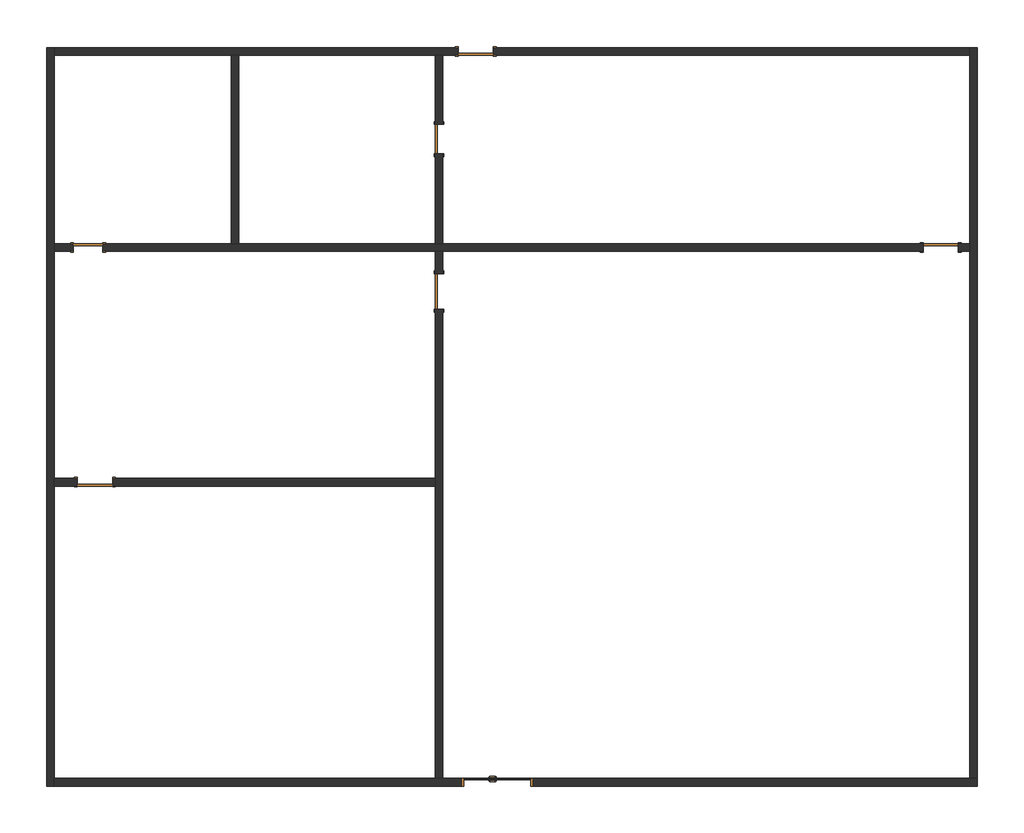
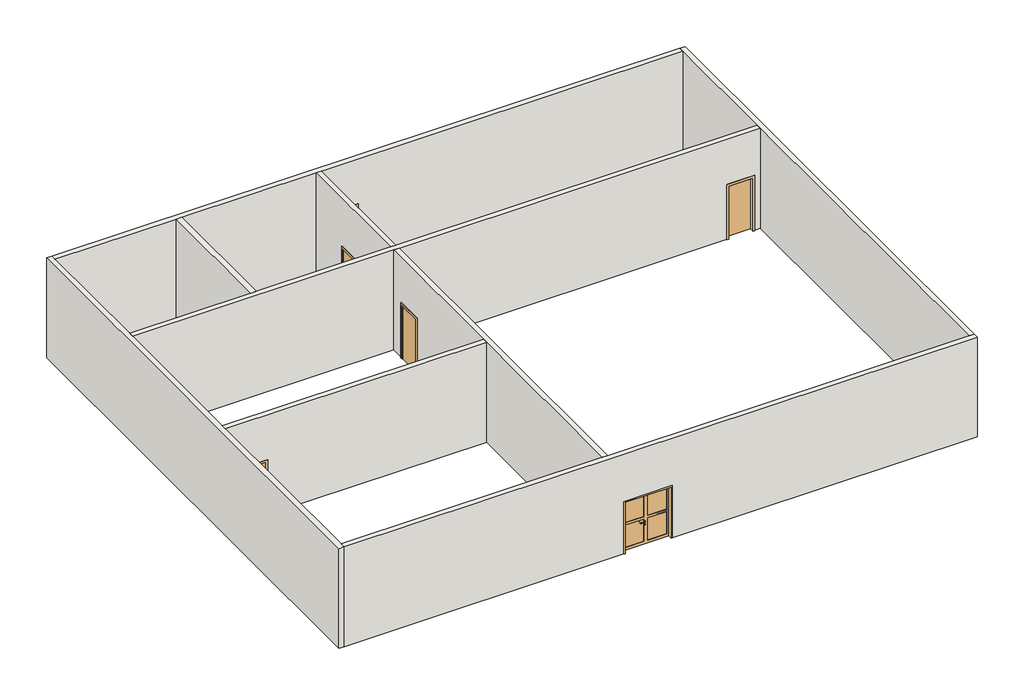
# One storey: 8 walls, 7 doors.
"""IFC4 building model written with IfcOpenShell, lengths in millimetres."""

import ifcopenshell
import ifcopenshell.guid

model = None  # the IFC model being written
_history = None  # IfcOwnerHistory: only IFC2X3 demands one
_inside = {}  # id of a spatial element -> (the spatial element, [elements in it])
_under = {}  # id of a project, library or spatial element -> (it, [spatial elements below it])
_declared = {}  # id of a project -> (the project, [libraries it declares])
_typed = {}  # id of a type object -> (the type object, [elements of that type])
_made_of = {}  # id of a material, layer set ... -> (it, [elements and type objects made of it])


def new_model(schema):
    """Start an empty IFC model of exactly this schema.

    Asked for "IFC4X3", IfcOpenShell would pick the latest addendum, in which some entities
    have other attributes; the version numbers below select the first issue.
    IFC2X3 requires an IfcOwnerHistory on every rooted entity: one is made here for all.
    """
    global model, _history
    if schema == "IFC4X3":
        model = ifcopenshell.file(schema_version=(4, 3, 0, 0))
    else:
        model = ifcopenshell.file(schema=schema)
    _inside.clear()
    _under.clear()
    _declared.clear()
    _typed.clear()
    _made_of.clear()
    _history = None
    if model.schema == "IFC2X3":
        org = make("IfcOrganization", Name="unknown")
        user = make(
            "IfcPersonAndOrganization",
            ThePerson=make("IfcPerson", FamilyName="unknown"),
            TheOrganization=org,
        )
        app = make(
            "IfcApplication",
            ApplicationDeveloper=org,
            Version="unknown",
            ApplicationFullName="unknown",
            ApplicationIdentifier="unknown",
        )
        _history = make(
            "IfcOwnerHistory",
            OwningUser=user,
            OwningApplication=app,
            ChangeAction="ADDED",
            CreationDate=0,
        )
    return model


def make(cls, **values):
    """One entity of the class cls with the attributes given. An attribute that is None is left unset."""
    return model.create_entity(
        cls, **{name: value for name, value in values.items() if value is not None}
    )


def rooted(cls, **values):
    """An entity with a GlobalId (a new one), such as an element, a storey or a relation."""
    return make(cls, GlobalId=ifcopenshell.guid.new(), OwnerHistory=_history, **values)


def si_unit(unit_type, name, prefix=None):
    """IfcSIUnit, for example si_unit("LENGTHUNIT", "METRE", prefix="MILLI")."""
    return make("IfcSIUnit", UnitType=unit_type, Prefix=prefix, Name=name)


def assignment(units):
    """IfcUnitAssignment: the units of a project."""
    return None if units is None else make("IfcUnitAssignment", Units=units)


def point(xyz):
    """IfcCartesianPoint."""
    return None if xyz is None else make("IfcCartesianPoint", Coordinates=xyz)


def direction(xyz):
    """IfcDirection."""
    return None if xyz is None else make("IfcDirection", DirectionRatios=xyz)


def frame(location, z_axis=None, x_axis=None):
    """IfcAxis2Placement3D, a coordinate frame: its origin and axes. An axis left out is left unset."""
    return make(
        "IfcAxis2Placement3D",
        Location=point(location),
        Axis=direction(z_axis),
        RefDirection=direction(x_axis),
    )


def frame_2d(location, x_axis=None):
    """IfcAxis2Placement2D, a coordinate frame in the plane: its origin and x axis."""
    return make(
        "IfcAxis2Placement2D", Location=point(location), RefDirection=direction(x_axis)
    )


def origin():
    """The frame at (0, 0, 0) with its axes left unset."""
    return frame((0.0, 0.0, 0.0))


def origin_with_axes():
    """The frame at (0, 0, 0) with the z axis (0, 0, 1) and the x axis (1, 0, 0) written out."""
    return frame((0.0, 0.0, 0.0), z_axis=(0.0, 0.0, 1.0), x_axis=(1.0, 0.0, 0.0))


def place(relative_to, where):
    """IfcLocalPlacement: puts the frame where relative to a parent placement (None: the world)."""
    return make(
        "IfcLocalPlacement", PlacementRelTo=relative_to, RelativePlacement=where
    )


def context(
    kind, dimensions, precision=None, world=None, true_north=None, identifier=None
):
    """IfcGeometricRepresentationContext, for example the 3D "Model" context."""
    return make(
        "IfcGeometricRepresentationContext",
        ContextIdentifier=identifier,
        ContextType=kind,
        CoordinateSpaceDimension=dimensions,
        Precision=precision,
        WorldCoordinateSystem=world,
        TrueNorth=true_north,
    )


def project(units=None, contexts=None):
    """IfcProject with its units and contexts."""
    return rooted(
        "IfcProject",
        Name="project",
        RepresentationContexts=contexts,
        UnitsInContext=assignment(units),
    )


def spatial(cls, under=None, at=None, **own):
    """A site, building, storey or space (cls), placed at a placement, below another one or the project."""
    s = rooted(cls, ObjectPlacement=at, **own)
    if under is not None:
        _under.setdefault(under.id(), (under, []))[1].append(s)
    return s


def polyline(points):
    """IfcPolyline through the points."""
    return make("IfcPolyline", Points=[point(p) for p in points])


def circle_curve(where, radius):
    """IfcCircle in the frame where."""
    return make("IfcCircle", Position=where, Radius=radius)


def ellipse_curve(where, semi_axis1, semi_axis2):
    """IfcEllipse in the frame where."""
    return make(
        "IfcEllipse", Position=where, SemiAxis1=semi_axis1, SemiAxis2=semi_axis2
    )


def trimmed(basis, trim1, trim2, sense, master):
    """IfcTrimmedCurve: the piece of a basis curve between two trims."""
    return make(
        "IfcTrimmedCurve",
        BasisCurve=basis,
        Trim1=trim1,
        Trim2=trim2,
        SenseAgreement=sense,
        MasterRepresentation=master,
    )


def segment(curve, same_sense, transition):
    """IfcCompositeCurveSegment."""
    return make(
        "IfcCompositeCurveSegment",
        Transition=transition,
        SameSense=same_sense,
        ParentCurve=curve,
    )


def composite_curve(segments, self_intersect=None):
    """IfcCompositeCurve: segments joined end to end."""
    return make("IfcCompositeCurve", Segments=segments, SelfIntersect=self_intersect)


def outline(outer, holes=None, kind="AREA"):
    """IfcArbitraryClosedProfileDef: a profile drawn as a closed curve; with holes, ...WithVoids."""
    if holes is None:
        return make("IfcArbitraryClosedProfileDef", ProfileType=kind, OuterCurve=outer)
    return make(
        "IfcArbitraryProfileDefWithVoids",
        ProfileType=kind,
        OuterCurve=outer,
        InnerCurves=holes,
    )


def extrude(swept, where, along, depth):
    """IfcExtrudedAreaSolid: the profile swept, set in the frame where, extruded along a direction by depth."""
    return make(
        "IfcExtrudedAreaSolid",
        SweptArea=swept,
        Position=where,
        ExtrudedDirection=direction(along),
        Depth=depth,
    )


def faces_of(points, faces, orient=None, outer=None):
    """IfcFace entities. A face is a list of loops; a loop is a list of indices into points, from 0.

    orient and outer hold one flag for each loop. By default every Orientation is true, the
    first loop of a face is its IfcFaceOuterBound and the others are IfcFaceBound.
    """
    made = []
    for i, loops in enumerate(faces):
        bounds = []
        for j, loop in enumerate(loops):
            is_outer = j == 0 if outer is None else outer[i][j]
            bounds.append(
                make(
                    "IfcFaceOuterBound" if is_outer else "IfcFaceBound",
                    Bound=make("IfcPolyLoop", Polygon=[points[k] for k in loop]),
                    Orientation=True if orient is None else orient[i][j],
                )
            )
        made.append(make("IfcFace", Bounds=bounds))
    return made


def faceted_brep(points, faces, orient=None, outer=None, voids=None):
    """IfcFacetedBrep: a solid bounded by flat faces; with voids (closed shells), ...WithVoids."""
    shared = [point(p) for p in points]
    hull = make("IfcClosedShell", CfsFaces=faces_of(shared, faces, orient, outer))
    if voids is None:
        return make("IfcFacetedBrep", Outer=hull)
    return make(
        "IfcFacetedBrepWithVoids",
        Outer=hull,
        Voids=[
            make(cls, CfsFaces=faces_of(shared, fs, o, b)) for cls, fs, o, b in voids
        ],
    )


def shape(context_of_items, identifier, shape_type, items):
    """IfcShapeRepresentation: the items that make up one representation, for example the "Body"."""
    return make(
        "IfcShapeRepresentation",
        ContextOfItems=context_of_items,
        RepresentationIdentifier=identifier,
        RepresentationType=shape_type,
        Items=items,
    )


def source(mapping_origin, context_of_items, identifier, shape_type, items):
    """IfcRepresentationMap: a shape defined once, which mapped items show again and again."""
    return make(
        "IfcRepresentationMap",
        MappingOrigin=mapping_origin,
        MappedRepresentation=shape(context_of_items, identifier, shape_type, items),
    )


def transform(
    local_origin,
    x_axis=None,
    y_axis=None,
    z_axis=None,
    scale=None,
    scale2=None,
    scale3=None,
    uniform=True,
):
    """IfcCartesianTransformationOperator3D, or its non-uniform kind. x_axis, y_axis, z_axis: its Axis1, 2, 3."""
    if uniform:
        return make(
            "IfcCartesianTransformationOperator3D",
            Axis1=direction(x_axis),
            Axis2=direction(y_axis),
            LocalOrigin=point(local_origin),
            Scale=scale,
            Axis3=direction(z_axis),
        )
    return make(
        "IfcCartesianTransformationOperator3DnonUniform",
        Axis1=direction(x_axis),
        Axis2=direction(y_axis),
        LocalOrigin=point(local_origin),
        Scale=scale,
        Axis3=direction(z_axis),
        Scale2=scale2,
        Scale3=scale3,
    )


def mapped(mapping_source, mapping_target):
    """IfcMappedItem: shows the shape of a source again, moved by a transform."""
    return make(
        "IfcMappedItem", MappingSource=mapping_source, MappingTarget=mapping_target
    )


def made_of(thing, what):
    """Note that an element or type object is made of a material, layer set ...; save() writes the relation."""
    if what is not None:
        _made_of.setdefault(what.id(), (what, []))[1].append(thing)
    return thing


def element(
    cls,
    number,
    at=None,
    inside=None,
    cuts=None,
    type_object=None,
    material=None,
    context=None,
    identifier="Body",
    shape_type=None,
    held_by="IfcProductDefinitionShape",
    body=None,
    shapes=None,
    **own,
):
    """One element of the class cls, such as IfcWall. Its Tag is "e" and its number.

    at: its placement. inside: the storey or other place that contains it. cuts: it is an
    opening in that element (IfcRelVoidsElement). A single representation is given by context,
    identifier, shape_type and body (its items); several are given by shapes. held_by: the class
    of the entity that holds the representations. save() writes the other relations.
    """
    e = rooted(cls, Tag="e%d" % number, ObjectPlacement=at, **own)
    if body is not None:
        shapes = [shape(context, identifier, shape_type, body)]
    if shapes is not None:
        e.Representation = make(held_by, Representations=shapes)
    if inside is not None:
        _inside.setdefault(inside.id(), (inside, []))[1].append(e)
    if cuts is not None:
        rooted(
            "IfcRelVoidsElement", RelatingBuildingElement=cuts, RelatedOpeningElement=e
        )
    if type_object is not None:
        _typed.setdefault(type_object.id(), (type_object, []))[1].append(e)
    return made_of(e, material)


def aggregate(whole, parts):
    """IfcRelAggregates: a whole, such as a stair, and the parts it consists of."""
    return rooted("IfcRelAggregates", RelatingObject=whole, RelatedObjects=parts)


def save(model, path):
    """Write the relations noted so far, then the file.

    IfcRelAggregates (storeys below a building ...), IfcRelContainedInSpatialStructure (elements
    in a storey), IfcRelDefinesByType, IfcRelAssociatesMaterial and IfcRelDeclares: one each for
    every whole, place, type object, material and project.
    """
    for whole, parts in _under.values():
        aggregate(whole, parts)
    for where, things in _inside.values():
        rooted(
            "IfcRelContainedInSpatialStructure",
            RelatedElements=things,
            RelatingStructure=where,
        )
    for kind, things in _typed.values():
        rooted("IfcRelDefinesByType", RelatedObjects=things, RelatingType=kind)
    for what, things in _made_of.values():
        rooted("IfcRelAssociatesMaterial", RelatedObjects=things, RelatingMaterial=what)
    for by, libraries in _declared.values():
        rooted("IfcRelDeclares", RelatingContext=by, RelatedDefinitions=libraries)
    model.write(path)


def plane_surface(at):
    """IfcPlane: the flat surface through the origin of the frame at, square to its z axis."""
    return make("IfcPlane", Position=at)


def cylinder_surface(at, radius):
    """IfcCylindricalSurface: all points at the distance radius from the z axis of the frame at."""
    return make("IfcCylindricalSurface", Position=at, Radius=radius)


def revolved_surface(curve, axis_point, axis_direction):
    """IfcSurfaceOfRevolution: the curve turned about the line through axis_point along axis_direction."""
    return make(
        "IfcSurfaceOfRevolution",
        SweptCurve=make("IfcArbitraryOpenProfileDef", ProfileType="CURVE", Curve=curve),
        AxisPosition=make("IfcAxis1Placement", Location=point(axis_point), Axis=direction(axis_direction)),
    )


def advanced_brep(points, edges, surfaces, faces):
    """IfcAdvancedBrep: a solid bounded by faces that lie on surfaces and meet in shared edges.

    An edge is (start, end): straight between two places in points (the first is 0);
    or (start, end, curve); or (start, end, curve, False) where it runs against its curve.
    A face is (place in surfaces, loops), or (place, loops, False) where it looks against
    its surface's normal. A loop lists edges by number (the first is 1), with a minus sign
    where the edge is run from its end to its start. The first loop is the outer one.
    """
    corners = [point(p) for p in points]
    vertices = [make("IfcVertexPoint", VertexGeometry=c) for c in corners]
    made = []
    for start, end, *more in edges:
        made.append(
            make(
                "IfcEdgeCurve",
                EdgeStart=vertices[start],
                EdgeEnd=vertices[end],
                EdgeGeometry=more[0] if more else make("IfcPolyline", Points=[corners[start], corners[end]]),
                SameSense=more[1] if len(more) > 1 else True,
            )
        )
    hull = []
    for where, loops, *sense in faces:
        bounds = []
        for j, loop in enumerate(loops):
            ring = [make("IfcOrientedEdge", EdgeElement=made[abs(k) - 1], Orientation=k > 0) for k in loop]
            bounds.append(
                make(
                    "IfcFaceOuterBound" if j == 0 else "IfcFaceBound",
                    Bound=make("IfcEdgeLoop", EdgeList=ring),
                    Orientation=True,
                )
            )
        hull.append(make("IfcAdvancedFace", Bounds=bounds, FaceSurface=surfaces[where], SameSense=sense[0] if sense else True))
    return make("IfcAdvancedBrep", Outer=make("IfcClosedShell", CfsFaces=hull))


def door_0762_x_2032mm_0c256fab(model_context):
    return source(origin(), model_context, "Body", "SweptSolid", [
        extrude(outline(polyline([(2108.0, -457.0), (0.0, -457.0), (0.0, -381.0), (2032.0, -381.0), (2032.0, 381.0), (0.0, 381.0), (0.0, 457.0), (2108.0, 457.0), (2108.0, -457.0)])), frame((0.0, 100.0, 0.0), z_axis=(0.0, 1.0, 0.0), x_axis=(0.0, 0.0, 1.0)), (0.0, 0.0, 1.0), 25.0),
        extrude(outline(polyline([(2108.0, 457.0), (2108.0, -457.0), (0.0, -457.0), (0.0, -381.0), (2032.0, -381.0), (2032.0, 381.0), (0.0, 381.0), (0.0, 457.0), (2108.0, 457.0)])), frame((0.0, -125.0, 0.0), z_axis=(0.0, 1.0, 0.0), x_axis=(0.0, 0.0, 1.0)), (0.0, 0.0, 1.0), 25.0),
        extrude(outline(polyline([(381.0, 49.0), (-381.0, 49.0), (-381.0, 100.0), (381.0, 100.0), (381.0, 49.0)])), origin_with_axes(), (0.0, 0.0, 1.0), 2032.0),
    ])


def door_0762_x_2032mm_7341a4fb(model_context):
    return source(origin(), model_context, "Body", "SweptSolid", [
        extrude(outline(polyline([(2108.0, -457.0), (0.0, -457.0), (0.0, -381.0), (2032.0, -381.0), (2032.0, 381.0), (0.0, 381.0), (0.0, 457.0), (2108.0, 457.0), (2108.0, -457.0)])), frame((0.0, -125.0, 0.0), z_axis=(0.0, 1.0, 0.0), x_axis=(0.0, 0.0, 1.0)), (0.0, 0.0, 1.0), 25.0),
        extrude(outline(polyline([(2108.0, 457.0), (2108.0, -457.0), (0.0, -457.0), (0.0, -381.0), (2032.0, -381.0), (2032.0, 381.0), (0.0, 381.0), (0.0, 457.0), (2108.0, 457.0)])), frame((0.0, 100.0, 0.0), z_axis=(0.0, 1.0, 0.0), x_axis=(0.0, 0.0, 1.0)), (0.0, 0.0, 1.0), 25.0),
        extrude(outline(polyline([(381.0, -49.0), (381.0, -100.0), (-381.0, -100.0), (-381.0, -49.0), (381.0, -49.0)])), origin_with_axes(), (0.0, 0.0, 1.0), 2032.0),
    ])


def door_0915_x_2134mm_6a9e8738(model_context):
    return source(origin(), model_context, "Body", "SweptSolid", [
        extrude(outline(polyline([(2210.0, -533.5), (0.0, -533.5), (0.0, -457.5), (2134.0, -457.5), (2134.0, 457.5), (0.0, 457.5), (0.0, 533.5), (2210.0, 533.5), (2210.0, -533.5)])), frame((0.0, 100.0, 0.0), z_axis=(0.0, 1.0, 0.0), x_axis=(0.0, 0.0, 1.0)), (0.0, 0.0, 1.0), 25.0),
        extrude(outline(polyline([(2210.0, 533.5), (2210.0, -533.5), (0.0, -533.5), (0.0, -457.5), (2134.0, -457.5), (2134.0, 457.5), (0.0, 457.5), (0.0, 533.5), (2210.0, 533.5)])), frame((0.0, -125.0, 0.0), z_axis=(0.0, 1.0, 0.0), x_axis=(0.0, 0.0, 1.0)), (0.0, 0.0, 1.0), 25.0),
        extrude(outline(polyline([(457.5, 49.0), (-457.5, 49.0), (-457.5, 100.0), (457.5, 100.0), (457.5, 49.0)])), origin_with_axes(), (0.0, 0.0, 1.0), 2134.0),
    ])


def porta_de_entrada_dupla_sem_revestimento_1840_x_2100mm_60e580c7(model_context):
    return source(origin(), model_context, "Body", "SolidModel", [
        advanced_brep(
        [(52.0, -57.0, 900.0), (28.0, -57.0, 900.0), (52.0, -40.0, 900.0), (28.0, -40.0, 900.0), (55.0, -13.0, 900.0), (55.0, -37.0, 900.0), (195.0, -37.0, 900.0), (195.0, -13.0, 900.0), (222.0, -40.0, 900.0), (198.0, -40.0, 900.0), (198.0, -55.0, 900.0), (222.0, -55.0, 900.0)],
        [
            (0, 1, circle_curve(frame((40.0, -57.0, 900.0), z_axis=(0.0, -1.0, 0.0), x_axis=(-1.0, 0.0, 0.0)), 12.0)),
            (1, 0, circle_curve(frame((40.0, -57.0, 900.0), z_axis=(0.0, -1.0, 0.0), x_axis=(-1.0, 0.0, 0.0)), 12.0)),
            (0, 2),
            (2, 3, circle_curve(frame((40.0, -40.0, 900.0), z_axis=(0.0, -1.0, 0.0), x_axis=(-1.0, 0.0, 0.0)), 12.0)),
            (3, 1),
            (3, 2, circle_curve(frame((40.0, -40.0, 900.0), z_axis=(0.0, -1.0, 0.0), x_axis=(-1.0, 0.0, 0.0)), 12.0)),
            (4, 3, circle_curve(frame((55.0, -40.0, 900.0), z_axis=(0.0, 0.0, 1.0), x_axis=(-1.0, 0.0, 0.0)), 27.0)),
            (2, 5, circle_curve(frame((55.0, -40.0, 900.0), z_axis=(0.0, 0.0, -1.0), x_axis=(-1.0, 0.0, 0.0)), 3.0)),
            (5, 4, circle_curve(frame((55.0, -25.0, 900.0), z_axis=(-1.0, 0.0, 0.0), x_axis=(0.0, 1.0, 0.0)), 12.0)),
            (4, 5, circle_curve(frame((55.0, -25.0, 900.0), z_axis=(-1.0, 0.0, 0.0), x_axis=(0.0, 1.0, 0.0)), 12.0)),
            (5, 6),
            (6, 7, circle_curve(frame((195.0, -25.0, 900.0), z_axis=(-1.0, 0.0, 0.0), x_axis=(0.0, 1.0, 0.0)), 12.0)),
            (7, 4),
            (7, 6, circle_curve(frame((195.0, -25.0, 900.0), z_axis=(-1.0, 0.0, 0.0), x_axis=(0.0, 1.0, 0.0)), 12.0)),
            (8, 7, circle_curve(frame((195.0, -40.0, 900.0), z_axis=(0.0, 0.0, 1.0), x_axis=(0.0, 1.0, 0.0)), 27.0)),
            (6, 9, circle_curve(frame((195.0, -40.0, 900.0), z_axis=(0.0, 0.0, -1.0), x_axis=(0.0, 1.0, 0.0)), 3.0)),
            (9, 8, circle_curve(frame((210.0, -40.0, 900.0), z_axis=(0.0, 1.0, 0.0), x_axis=(1.0, 0.0, 0.0)), 12.0)),
            (8, 9, circle_curve(frame((210.0, -40.0, 900.0), z_axis=(0.0, 1.0, 0.0), x_axis=(1.0, 0.0, 0.0)), 12.0)),
            (10, 11, circle_curve(frame((210.0, -55.0, 900.0), z_axis=(0.0, -1.0, 0.0), x_axis=(1.0, 0.0, 0.0)), 12.0)),
            (11, 10, circle_curve(frame((210.0, -55.0, 900.0), z_axis=(0.0, -1.0, 0.0), x_axis=(1.0, 0.0, 0.0)), 12.0)),
            (9, 10),
            (11, 8),
        ],
        [
            plane_surface(frame((-802.0, -57.0, 1730.0), z_axis=(0.0, -1.0, 0.0), x_axis=(0.0, 0.0, 1.0))),
            cylinder_surface(frame((40.0, -57.0, 900.0), z_axis=(0.0, -1.0, 0.0), x_axis=(-1.0, 0.0, 0.0)), 12.0),
            revolved_surface(trimmed(ellipse_curve(frame((40.0, -40.0, 900.0), z_axis=(0.0, -1.0, 0.0), x_axis=(-1.0, 0.0, 0.0)), 12.0, 12.0), [point((52.0, -40.0, 900.0))], [point((28.0, -40.0, 900.0))], True, "CARTESIAN"), (55.0, -40.0, 1730.0), (0.0, 0.0, -1.0)),
            revolved_surface(trimmed(ellipse_curve(frame((40.0, -40.0, 900.0), z_axis=(0.0, -1.0, 0.0), x_axis=(-1.0, 0.0, 0.0)), 12.0, 12.0), [point((28.0, -40.0, 900.0))], [point((52.0, -40.0, 900.0))], True, "CARTESIAN"), (55.0, -40.0, 1730.0), (0.0, 0.0, -1.0)),
            cylinder_surface(frame((55.0, -25.0, 900.0), z_axis=(-1.0, 0.0, 0.0), x_axis=(0.0, 1.0, 0.0)), 12.0),
            revolved_surface(trimmed(ellipse_curve(frame((195.0, -25.0, 900.0), z_axis=(-1.0, 0.0, 0.0), x_axis=(0.0, 1.0, 0.0)), 12.0, 12.0), [point((195.0, -37.0, 900.0))], [point((195.0, -13.0, 900.0))], True, "CARTESIAN"), (195.0, -40.0, 1730.0), (0.0, 0.0, -1.0)),
            revolved_surface(trimmed(ellipse_curve(frame((195.0, -25.0, 900.0), z_axis=(-1.0, 0.0, 0.0), x_axis=(0.0, 1.0, 0.0)), 12.0, 12.0), [point((195.0, -13.0, 900.0))], [point((195.0, -37.0, 900.0))], True, "CARTESIAN"), (195.0, -40.0, 1730.0), (0.0, 0.0, -1.0)),
            plane_surface(frame((-632.0, -55.0, 1730.0), z_axis=(0.0, -1.0, 0.0), x_axis=(0.0, 0.0, -1.0))),
            cylinder_surface(frame((210.0, -40.0, 900.0), z_axis=(0.0, 1.0, 0.0), x_axis=(1.0, 0.0, 0.0)), 12.0),
        ],
        [
            (0, [[1, 2]]),
            (1, [[-1, 3, 4, 5]]),
            (1, [[-2, -5, 6, -3]]),
            (2, [[7, -4, 8, 9]]),
            (3, [[-8, -6, -7, 10]]),
            (4, [[-9, 11, 12, 13]]),
            (4, [[-10, -13, 14, -11]]),
            (5, [[15, -12, 16, 17]]),
            (6, [[-16, -14, -15, 18]]),
            (7, [[19, 20]]),
            (8, [[-17, 21, -20, 22]]),
            (8, [[-18, -22, -19, -21]]),
        ],
    ),
        extrude(outline(composite_curve([segment(trimmed(circle_curve(frame_2d((780.0, 40.0)), 25.0), [point((780.0, 15.0))], [point((780.0, 65.0))], False, "CARTESIAN"), True, "CONTINUOUS"), segment(trimmed(circle_curve(frame_2d((780.0, 40.0)), 25.0), [point((780.0, 65.0))], [point((780.0, 15.0))], False, "CARTESIAN"), True, "CONTINUOUS")], self_intersect=False)), frame((0.0, -65.0, 0.0), z_axis=(0.0, 1.0, 0.0), x_axis=(0.0, 0.0, 1.0)), (0.0, 0.0, 1.0), 8.0),
        extrude(outline(composite_curve([segment(trimmed(circle_curve(frame_2d((900.0, 40.0)), 25.0), [point((900.0, 15.0))], [point((900.0, 65.0))], False, "CARTESIAN"), True, "CONTINUOUS"), segment(trimmed(circle_curve(frame_2d((900.0, 40.0)), 25.0), [point((900.0, 65.0))], [point((900.0, 15.0))], False, "CARTESIAN"), True, "CONTINUOUS")], self_intersect=False)), frame((0.0, -65.0, 0.0), z_axis=(0.0, 1.0, 0.0), x_axis=(0.0, 0.0, 1.0)), (0.0, 0.0, 1.0), 8.0),
        advanced_brep(
        [(28.0, -108.0, 900.0), (52.0, -108.0, 900.0), (28.0, -125.0, 900.0), (52.0, -125.0, 900.0), (55.0, -128.0, 900.0), (55.0, -152.0, 900.0), (195.0, -152.0, 900.0), (195.0, -128.0, 900.0), (198.0, -125.0, 900.0), (222.0, -125.0, 900.0), (222.0, -110.0, 900.0), (198.0, -110.0, 900.0)],
        [
            (0, 1, circle_curve(frame((40.0, -108.0, 900.0), z_axis=(0.0, 1.0, 0.0), x_axis=(1.0, 0.0, 0.0)), 12.0)),
            (1, 0, circle_curve(frame((40.0, -108.0, 900.0), z_axis=(0.0, 1.0, 0.0), x_axis=(1.0, 0.0, 0.0)), 12.0)),
            (0, 2),
            (2, 3, circle_curve(frame((40.0, -125.0, 900.0), z_axis=(0.0, 1.0, 0.0), x_axis=(1.0, 0.0, 0.0)), 12.0)),
            (3, 1),
            (3, 2, circle_curve(frame((40.0, -125.0, 900.0), z_axis=(0.0, 1.0, 0.0), x_axis=(1.0, 0.0, 0.0)), 12.0)),
            (4, 3, circle_curve(frame((55.0, -125.0, 900.0), z_axis=(0.0, 0.0, -1.0), x_axis=(-1.0, 0.0, 0.0)), 3.0)),
            (2, 5, circle_curve(frame((55.0, -125.0, 900.0), z_axis=(0.0, 0.0, 1.0), x_axis=(-1.0, 0.0, 0.0)), 27.0)),
            (5, 4, circle_curve(frame((55.0, -140.0, 900.0), z_axis=(-1.0, 0.0, 0.0), x_axis=(0.0, 1.0, 0.0)), 12.0)),
            (4, 5, circle_curve(frame((55.0, -140.0, 900.0), z_axis=(-1.0, 0.0, 0.0), x_axis=(0.0, 1.0, 0.0)), 12.0)),
            (5, 6),
            (6, 7, circle_curve(frame((195.0, -140.0, 900.0), z_axis=(-1.0, 0.0, 0.0), x_axis=(0.0, 1.0, 0.0)), 12.0)),
            (7, 4),
            (7, 6, circle_curve(frame((195.0, -140.0, 900.0), z_axis=(-1.0, 0.0, 0.0), x_axis=(0.0, 1.0, 0.0)), 12.0)),
            (8, 7, circle_curve(frame((195.0, -125.0, 900.0), z_axis=(0.0, 0.0, -1.0), x_axis=(0.0, -1.0, 0.0)), 3.0)),
            (6, 9, circle_curve(frame((195.0, -125.0, 900.0), z_axis=(0.0, 0.0, 1.0), x_axis=(0.0, -1.0, 0.0)), 27.0)),
            (9, 8, circle_curve(frame((210.0, -125.0, 900.0), z_axis=(0.0, -1.0, 0.0), x_axis=(-1.0, 0.0, 0.0)), 12.0)),
            (8, 9, circle_curve(frame((210.0, -125.0, 900.0), z_axis=(0.0, -1.0, 0.0), x_axis=(-1.0, 0.0, 0.0)), 12.0)),
            (10, 11, circle_curve(frame((210.0, -110.0, 900.0), z_axis=(0.0, 1.0, 0.0), x_axis=(-1.0, 0.0, 0.0)), 12.0)),
            (11, 10, circle_curve(frame((210.0, -110.0, 900.0), z_axis=(0.0, 1.0, 0.0), x_axis=(-1.0, 0.0, 0.0)), 12.0)),
            (9, 10),
            (11, 8),
        ],
        [
            plane_surface(frame((-802.0, -108.0, 1730.0), z_axis=(0.0, 1.0, 0.0), x_axis=(0.0, 0.0, -1.0))),
            cylinder_surface(frame((40.0, -108.0, 900.0), z_axis=(0.0, 1.0, 0.0), x_axis=(1.0, 0.0, 0.0)), 12.0),
            revolved_surface(trimmed(ellipse_curve(frame((40.0, -125.0, 900.0), z_axis=(0.0, 1.0, 0.0), x_axis=(1.0, 0.0, 0.0)), 12.0, 12.0), [point((28.0, -125.0, 900.0))], [point((52.0, -125.0, 900.0))], True, "CARTESIAN"), (55.0, -125.0, 1730.0), (0.0, 0.0, 1.0)),
            revolved_surface(trimmed(ellipse_curve(frame((40.0, -125.0, 900.0), z_axis=(0.0, 1.0, 0.0), x_axis=(1.0, 0.0, 0.0)), 12.0, 12.0), [point((52.0, -125.0, 900.0))], [point((28.0, -125.0, 900.0))], True, "CARTESIAN"), (55.0, -125.0, 1730.0), (0.0, 0.0, 1.0)),
            cylinder_surface(frame((55.0, -140.0, 900.0), z_axis=(-1.0, 0.0, 0.0), x_axis=(0.0, 1.0, 0.0)), 12.0),
            revolved_surface(trimmed(ellipse_curve(frame((195.0, -140.0, 900.0), z_axis=(-1.0, 0.0, 0.0), x_axis=(0.0, 1.0, 0.0)), 12.0, 12.0), [point((195.0, -152.0, 900.0))], [point((195.0, -128.0, 900.0))], True, "CARTESIAN"), (195.0, -125.0, 1730.0), (0.0, 0.0, 1.0)),
            revolved_surface(trimmed(ellipse_curve(frame((195.0, -140.0, 900.0), z_axis=(-1.0, 0.0, 0.0), x_axis=(0.0, 1.0, 0.0)), 12.0, 12.0), [point((195.0, -128.0, 900.0))], [point((195.0, -152.0, 900.0))], True, "CARTESIAN"), (195.0, -125.0, 1730.0), (0.0, 0.0, 1.0)),
            plane_surface(frame((-632.0, -110.0, 1730.0), z_axis=(0.0, 1.0, 0.0), x_axis=(0.0, 0.0, 1.0))),
            cylinder_surface(frame((210.0, -125.0, 900.0), z_axis=(0.0, -1.0, 0.0), x_axis=(-1.0, 0.0, 0.0)), 12.0),
        ],
        [
            (0, [[1, 2]]),
            (1, [[-1, 3, 4, 5]]),
            (1, [[-2, -5, 6, -3]]),
            (2, [[7, -4, 8, 9]]),
            (3, [[-8, -6, -7, 10]]),
            (4, [[-9, 11, 12, 13]]),
            (4, [[-10, -13, 14, -11]]),
            (5, [[15, -12, 16, 17]]),
            (6, [[-16, -14, -15, 18]]),
            (7, [[19, 20]]),
            (8, [[-17, 21, -20, 22]]),
            (8, [[-18, -22, -19, -21]]),
        ],
    ),
        extrude(outline(composite_curve([segment(trimmed(circle_curve(frame_2d((780.0, 40.0)), 25.0), [point((780.0, 15.0))], [point((780.0, 65.0))], False, "CARTESIAN"), True, "CONTINUOUS"), segment(trimmed(circle_curve(frame_2d((780.0, 40.0)), 25.0), [point((780.0, 65.0))], [point((780.0, 15.0))], False, "CARTESIAN"), True, "CONTINUOUS")], self_intersect=False)), frame((0.0, -108.0, 0.0), z_axis=(0.0, 1.0, 0.0), x_axis=(0.0, 0.0, 1.0)), (0.0, 0.0, 1.0), 8.0),
        extrude(outline(composite_curve([segment(trimmed(circle_curve(frame_2d((900.0, 40.0)), 25.0), [point((900.0, 15.0))], [point((900.0, 65.0))], False, "CARTESIAN"), True, "CONTINUOUS"), segment(trimmed(circle_curve(frame_2d((900.0, 40.0)), 25.0), [point((900.0, 65.0))], [point((900.0, 15.0))], False, "CARTESIAN"), True, "CONTINUOUS")], self_intersect=False)), frame((0.0, -108.0, 0.0), z_axis=(0.0, 1.0, 0.0), x_axis=(0.0, 0.0, 1.0)), (0.0, 0.0, 1.0), 8.0),
        extrude(outline(polyline([(-835.0, -75.5), (835.0, -75.5), (835.0, -89.5), (-835.0, -89.5), (-835.0, -75.5)])), frame((0.0, 0.0, 70.0), z_axis=(0.0, 0.0, 1.0), x_axis=(1.0, 0.0, 0.0)), (0.0, 0.0, 1.0), 970.0),
        extrude(outline(polyline([(-835.0, -75.5), (835.0, -75.5), (835.0, -89.5), (-835.0, -89.5), (-835.0, -75.5)])), frame((0.0, 0.0, 1060.0), z_axis=(0.0, 0.0, 1.0), x_axis=(1.0, 0.0, 0.0)), (0.0, 0.0, 1.0), 955.0),
        extrude(outline(polyline([(-835.0, -75.5), (835.0, -75.5), (835.0, -89.5), (-835.0, -89.5), (-835.0, -75.5)])), frame((0.0, 0.0, 70.0), z_axis=(0.0, 0.0, 1.0), x_axis=(1.0, 0.0, 0.0)), (0.0, 0.0, 1.0), 970.0),
        extrude(outline(polyline([(-835.0, -75.5), (835.0, -75.5), (835.0, -89.5), (-835.0, -89.5), (-835.0, -75.5)])), frame((0.0, 0.0, 1060.0), z_axis=(0.0, 0.0, 1.0), x_axis=(1.0, 0.0, 0.0)), (0.0, 0.0, 1.0), 955.0),
        faceted_brep([(-920.0, 100.0, 0.0), (-870.0, 100.0, 0.0), (-870.0, -62.0, 0.0), (-880.0, -62.0, 0.0), (-880.0, -100.0, 0.0), (-920.0, -100.0, 0.0), (-920.0, 100.0, 2100.0), (920.0, 100.0, 2100.0), (920.0, 100.0, 0.0), (870.0, 100.0, 0.0), (870.0, 100.0, 2050.0), (-870.0, 100.0, 2050.0), (-870.0, -62.0, 2050.0), (870.0, -62.0, 2050.0), (870.0, -62.0, 0.0), (880.0, -62.0, 0.0), (880.0, -62.0, 2060.0), (-880.0, -62.0, 2060.0), (-880.0, -100.0, 2060.0), (880.0, -100.0, 2060.0), (880.0, -100.0, 0.0), (920.0, -100.0, 0.0), (920.0, -100.0, 2100.0), (-920.0, -100.0, 2100.0)], [[[0, 1, 2, 3, 4, 5]], [[1, 0, 6, 7, 8, 9, 10, 11]], [[2, 1, 11, 12]], [[3, 2, 12, 13, 14, 15, 16, 17]], [[4, 3, 17, 18]], [[5, 4, 18, 19, 20, 21, 22, 23]], [[0, 5, 23, 6]], [[7, 22, 21, 8]], [[8, 21, 20, 15, 14, 9]], [[13, 10, 9, 14]], [[19, 16, 15, 20]], [[12, 11, 10, 13]], [[18, 17, 16, 19]], [[6, 23, 22, 7]]]),
        extrude(outline(polyline([(2060.0, -880.0), (0.0, -880.0), (0.0, 880.0), (2060.0, 880.0), (2060.0, -880.0)]), holes=[polyline([(1975.0, 75.0), (1975.0, 795.0), (1100.0, 795.0), (1100.0, 75.0), (1975.0, 75.0)]), polyline([(1100.0, -795.0), (1975.0, -795.0), (1975.0, -75.0), (1100.0, -75.0), (1100.0, -795.0)]), polyline([(1000.0, 795.0), (110.0, 795.0), (110.0, 75.0), (1000.0, 75.0), (1000.0, 795.0)]), polyline([(110.0, -75.0), (110.0, -795.0), (1000.0, -795.0), (1000.0, -75.0), (110.0, -75.0)])]), frame((0.0, -100.0, 0.0), z_axis=(0.0, 1.0, 0.0), x_axis=(0.0, 0.0, 1.0)), (0.0, 0.0, 1.0), 35.0),
    ])


model = new_model("IFC4")

# Units and contexts
model_context = context("Model", 3, world=origin())
ifc_project = project(units=[si_unit("LENGTHUNIT", "METRE", prefix="MILLI")], contexts=[model_context])

# Site, building, storey
site = spatial("IfcSite", under=ifc_project)
building = spatial("IfcBuilding", under=site)
storey = spatial("IfcBuildingStorey", under=building, Name="Nível 1", Elevation=0.0)

# Doors
placement = place(None, origin())
door_0762_x_2032mm_shape = door_0762_x_2032mm_0c256fab(model_context)
element("IfcDoor", 1, ObjectType="M_Folha única : 0762 x 2032mm", at=placement, inside=storey, context=model_context, shape_type="MappedRepresentation", body=[
    mapped(door_0762_x_2032mm_shape, transform((-853.9170537, 8835.1002326, 0.0), x_axis=(0.0, 1.0, 0.0), y_axis=(-1.0, 0.0, 0.0), z_axis=(0.0, 0.0, 1.0))),
])
door_0762_x_2032mm_2_shape = door_0762_x_2032mm_7341a4fb(model_context)
element("IfcDoor", 2, ObjectType="M_Folha única : 0762 x 2032mm", at=placement, inside=storey, context=model_context, shape_type="MappedRepresentation", body=[
    mapped(door_0762_x_2032mm_2_shape, transform((-9972.9170537, 6016.1002326, 0.0), x_axis=(-1.0, 0.0, 0.0), y_axis=(0.0, -1.0, 0.0), z_axis=(0.0, 0.0, 1.0))),
])
door_0915_x_2134mm_shape = door_0915_x_2134mm_6a9e8738(model_context)
element("IfcDoor", 3, ObjectType="M_Folha única : 0915 x 2134mm", at=placement, inside=storey, context=model_context, shape_type="MappedRepresentation", body=[
    mapped(door_0915_x_2134mm_shape, transform((-853.9170537, 4873.6002326, 0.0), x_axis=(0.0, 1.0, 0.0), y_axis=(-1.0, 0.0, 0.0), z_axis=(0.0, 0.0, 1.0))),
])
element("IfcDoor", 4, ObjectType="M_Folha única : 0915 x 2134mm", at=placement, inside=storey, context=model_context, shape_type="MappedRepresentation", body=[
    mapped(door_0915_x_2134mm_shape, transform((103.5829463, 11116.1002326, 0.0), x_axis=(-1.0, 0.0, 0.0), y_axis=(0.0, -1.0, 0.0), z_axis=(0.0, 0.0, 1.0))),
])
element("IfcDoor", 5, ObjectType="M_Folha única : 0915 x 2134mm", at=placement, inside=storey, context=model_context, shape_type="MappedRepresentation", body=[
    mapped(door_0915_x_2134mm_shape, transform((-9796.4170537, -83.8997674, 0.0), x_axis=(-1.0, 0.0, 0.0), y_axis=(0.0, -1.0, 0.0), z_axis=(0.0, 0.0, 1.0))),
])
element("IfcDoor", 6, ObjectType="M_Folha única : 0915 x 2134mm", at=placement, inside=storey, context=model_context, shape_type="MappedRepresentation", body=[
    mapped(door_0915_x_2134mm_shape, transform((12188.5829463, 6016.1002326, 0.0), x_axis=(1.0, 0.0, 0.0), y_axis=(0.0, 1.0, 0.0), z_axis=(0.0, 0.0, 1.0))),
])
porta_de_entrada_dupla_sem_revestimento_1840_x_2100mm_shape = porta_de_entrada_dupla_sem_revestimento_1840_x_2100mm_60e580c7(model_context)
element("IfcDoor", 7, ObjectType="Porta de entrada dupla sem revestimento : 1840 x 2100mm", at=placement, inside=storey, context=model_context, shape_type="MappedRepresentation", body=[
    mapped(porta_de_entrada_dupla_sem_revestimento_1840_x_2100mm_shape, transform((666.0829463, -7883.8997674, 0.0), x_axis=(-1.0, 0.0, 0.0), y_axis=(0.0, -1.0, 0.0), z_axis=(0.0, 0.0, 1.0))),
])

# Walls
element("IfcWall", 8, ObjectType="Genérico - 200 mm", at=placement, inside=storey, context=model_context, shape_type="Brep", body=[
    faceted_brep([(-11053.9170537, 11216.1002326, 0.0), (-11053.9170537, -7983.8997674, 0.0), (-11053.9170537, -7983.8997674, 4000.0), (-11053.9170537, 11216.1002326, 4000.0), (-10853.9170537, 11216.1002326, 0.0), (-10853.9170537, 11216.1002326, 4000.0), (-10853.9170537, 11016.1002326, 4000.0), (-10853.9170537, 6116.1002326, 4000.0), (-10853.9170537, 5916.1002326, 4000.0), (-10853.9170537, 16.1002326, 4000.0), (-10853.9170537, -183.8997674, 4000.0), (-10853.9170537, -7783.8997674, 4000.0), (-10853.9170537, -7983.8997674, 4000.0), (-10853.9170537, -7983.8997674, 0.0), (-10853.9170537, -7783.8997674, 0.0), (-10853.9170537, -183.8997674, 0.0), (-10853.9170537, 16.1002326, 0.0), (-10853.9170537, 5916.1002326, 0.0), (-10853.9170537, 6116.1002326, 0.0), (-10853.9170537, 11016.1002326, 0.0)], [[[0, 1, 2, 3]], [[4, 5, 6, 7, 8, 9, 10, 11, 12, 13, 14, 15, 16, 17, 18, 19]], [[1, 0, 4, 19, 18, 17, 16, 15, 14, 13]], [[3, 2, 12, 11, 10, 9, 8, 7, 6, 5]], [[2, 1, 13, 12]], [[0, 3, 5, 4]]]),
])
element("IfcWall", 9, ObjectType="Genérico - 200 mm", at=placement, inside=storey, context=model_context, shape_type="Brep", body=[
    faceted_brep([(13146.0829463, -7983.8997674, 4000.0), (-10853.9170537, -7983.8997674, 4000.0), (-10853.9170537, -7983.8997674, 0.0), (-253.9170537, -7983.8997674, 0.0), (-253.9170537, -7983.8997674, 2100.0), (1586.0829463, -7983.8997674, 2100.0), (1586.0829463, -7983.8997674, 0.0), (13146.0829463, -7983.8997674, 0.0), (-10853.9170537, -7783.8997674, 4000.0), (-953.9170537, -7783.8997674, 4000.0), (-753.9170537, -7783.8997674, 4000.0), (12946.0829463, -7783.8997674, 4000.0), (13146.0829463, -7783.8997674, 4000.0), (13146.0829463, -7783.8997674, 0.0), (12946.0829463, -7783.8997674, 0.0), (1586.0829463, -7783.8997674, 0.0), (1586.0829463, -7783.8997674, 2100.0), (-253.9170537, -7783.8997674, 2100.0), (-253.9170537, -7783.8997674, 0.0), (-753.9170537, -7783.8997674, 0.0), (-953.9170537, -7783.8997674, 0.0), (-10853.9170537, -7783.8997674, 0.0)], [[[0, 1, 2, 3, 4, 5, 6, 7]], [[8, 9, 10, 11, 12, 13, 14, 15, 16, 17, 18, 19, 20, 21]], [[2, 21, 20, 19, 18, 3]], [[13, 7, 6, 15, 14]], [[1, 0, 12, 11, 10, 9, 8]], [[2, 1, 8, 21]], [[0, 7, 13, 12]], [[17, 4, 3, 18]], [[4, 17, 16, 5]], [[5, 16, 15, 6]]]),
])
element("IfcWall", 10, ObjectType="Genérico - 200 mm", at=placement, inside=storey, context=model_context, shape_type="Brep", body=[
    faceted_brep([(13146.0829463, -7783.8997674, 0.0), (13146.0829463, 11216.1002326, 0.0), (13146.0829463, 11216.1002326, 4000.0), (13146.0829463, -7783.8997674, 4000.0), (12946.0829463, -7783.8997674, 0.0), (12946.0829463, -7783.8997674, 4000.0), (12946.0829463, 5916.1002326, 4000.0), (12946.0829463, 6116.1002326, 4000.0), (12946.0829463, 11016.1002326, 4000.0), (12946.0829463, 11216.1002326, 4000.0), (12946.0829463, 11216.1002326, 0.0), (12946.0829463, 11016.1002326, 0.0), (12946.0829463, 6116.1002326, 0.0), (12946.0829463, 5916.1002326, 0.0)], [[[0, 1, 2, 3]], [[4, 5, 6, 7, 8, 9, 10, 11, 12, 13]], [[1, 0, 4, 13, 12, 11, 10]], [[3, 2, 9, 8, 7, 6, 5]], [[0, 3, 5, 4]], [[2, 1, 10, 9]]]),
])
element("IfcWall", 11, ObjectType="Genérico - 200 mm", at=placement, inside=storey, context=model_context, shape_type="Brep", body=[
    faceted_brep([(-353.9170537, 11216.1002326, 2134.0), (-353.9170537, 11216.1002326, 0.0), (-10853.9170537, 11216.1002326, 0.0), (-10853.9170537, 11216.1002326, 4000.0), (12946.0829463, 11216.1002326, 4000.0), (12946.0829463, 11216.1002326, 0.0), (561.0829463, 11216.1002326, 0.0), (561.0829463, 11216.1002326, 2134.0), (-10853.9170537, 11016.1002326, 0.0), (-6253.9170537, 11016.1002326, 0.0), (-6053.9170537, 11016.1002326, 0.0), (-953.9170537, 11016.1002326, 0.0), (-753.9170537, 11016.1002326, 0.0), (-353.9170537, 11016.1002326, 0.0), (-353.9170537, 11016.1002326, 2134.0), (561.0829463, 11016.1002326, 2134.0), (561.0829463, 11016.1002326, 0.0), (12946.0829463, 11016.1002326, 0.0), (12946.0829463, 11016.1002326, 4000.0), (-753.9170537, 11016.1002326, 4000.0), (-953.9170537, 11016.1002326, 4000.0), (-6053.9170537, 11016.1002326, 4000.0), (-6253.9170537, 11016.1002326, 4000.0), (-10853.9170537, 11016.1002326, 4000.0)], [[[0, 1, 2, 3, 4, 5, 6, 7]], [[8, 9, 10, 11, 12, 13, 14, 15, 16, 17, 18, 19, 20, 21, 22, 23]], [[6, 5, 17, 16]], [[2, 1, 13, 12, 11, 10, 9, 8]], [[4, 3, 23, 22, 21, 20, 19, 18]], [[3, 2, 8, 23]], [[5, 4, 18, 17]], [[14, 13, 1, 0]], [[15, 14, 0, 7]], [[16, 15, 7, 6]]]),
])
element("IfcWall", 12, ObjectType="Genérico - 200 mm", at=placement, inside=storey, context=model_context, shape_type="Brep", body=[
    faceted_brep([(-10853.9170537, 5916.1002326, 0.0), (-10353.9170537, 5916.1002326, 0.0), (-10353.9170537, 5916.1002326, 2032.0), (-9591.9170537, 5916.1002326, 2032.0), (-9591.9170537, 5916.1002326, 0.0), (-953.9170537, 5916.1002326, 0.0), (-753.9170537, 5916.1002326, 0.0), (11731.0829463, 5916.1002326, 0.0), (11731.0829463, 5916.1002326, 2134.0), (12646.0829463, 5916.1002326, 2134.0), (12646.0829463, 5916.1002326, 0.0), (12946.0829463, 5916.1002326, 0.0), (12946.0829463, 5916.1002326, 4000.0), (-753.9170537, 5916.1002326, 4000.0), (-953.9170537, 5916.1002326, 4000.0), (-10853.9170537, 5916.1002326, 4000.0), (-10353.9170537, 6116.1002326, 2032.0), (-10353.9170537, 6116.1002326, 0.0), (-10853.9170537, 6116.1002326, 0.0), (-10853.9170537, 6116.1002326, 4000.0), (-6253.9170537, 6116.1002326, 4000.0), (-6053.9170537, 6116.1002326, 4000.0), (-953.9170537, 6116.1002326, 4000.0), (-753.9170537, 6116.1002326, 4000.0), (12946.0829463, 6116.1002326, 4000.0), (12946.0829463, 6116.1002326, 0.0), (12646.0829463, 6116.1002326, 0.0), (12646.0829463, 6116.1002326, 2134.0), (11731.0829463, 6116.1002326, 2134.0), (11731.0829463, 6116.1002326, 0.0), (-753.9170537, 6116.1002326, 0.0), (-953.9170537, 6116.1002326, 0.0), (-6053.9170537, 6116.1002326, 0.0), (-6253.9170537, 6116.1002326, 0.0), (-9591.9170537, 6116.1002326, 0.0), (-9591.9170537, 6116.1002326, 2032.0)], [[[0, 1, 2, 3, 4, 5, 6, 7, 8, 9, 10, 11, 12, 13, 14, 15]], [[16, 17, 18, 19, 20, 21, 22, 23, 24, 25, 26, 27, 28, 29, 30, 31, 32, 33, 34, 35]], [[11, 10, 26, 25]], [[18, 17, 1, 0]], [[34, 33, 32, 31, 30, 29, 7, 6, 5, 4]], [[15, 14, 13, 12, 24, 23, 22, 21, 20, 19]], [[0, 15, 19, 18]], [[12, 11, 25, 24]], [[27, 26, 10, 9]], [[28, 27, 9, 8]], [[29, 28, 8, 7]], [[2, 1, 17, 16]], [[3, 2, 16, 35]], [[4, 3, 35, 34]]]),
])
element("IfcWall", 13, ObjectType="Genérico - 200 mm", at=placement, inside=storey, context=model_context, shape_type="Brep", body=[
    faceted_brep([(-953.9170537, -7783.8997674, 0.0), (-953.9170537, -7783.8997674, 4000.0), (-953.9170537, -183.8997674, 4000.0), (-953.9170537, 16.1002326, 4000.0), (-953.9170537, 5916.1002326, 4000.0), (-953.9170537, 5916.1002326, 0.0), (-953.9170537, 5331.1002326, 0.0), (-953.9170537, 5331.1002326, 2134.0), (-953.9170537, 4416.1002326, 2134.0), (-953.9170537, 4416.1002326, 0.0), (-953.9170537, 16.1002326, 0.0), (-953.9170537, -183.8997674, 0.0), (-753.9170537, -7783.8997674, 4000.0), (-753.9170537, -7783.8997674, 0.0), (-753.9170537, 4416.1002326, 0.0), (-753.9170537, 4416.1002326, 2134.0), (-753.9170537, 5331.1002326, 2134.0), (-753.9170537, 5331.1002326, 0.0), (-753.9170537, 5916.1002326, 0.0), (-753.9170537, 5916.1002326, 4000.0)], [[[0, 1, 2, 3, 4, 5, 6, 7, 8, 9, 10, 11]], [[12, 13, 14, 15, 16, 17, 18, 19]], [[13, 0, 11, 10, 9, 14]], [[17, 6, 5, 18]], [[1, 12, 19, 4, 3, 2]], [[1, 0, 13, 12]], [[5, 4, 19, 18]], [[7, 6, 17, 16]], [[8, 7, 16, 15]], [[9, 8, 15, 14]]]),
    faceted_brep([(-953.9170537, 11016.1002326, 4000.0), (-953.9170537, 11016.1002326, 0.0), (-953.9170537, 9216.1002326, 0.0), (-953.9170537, 9216.1002326, 2032.0), (-953.9170537, 8454.1002326, 2032.0), (-953.9170537, 8454.1002326, 0.0), (-953.9170537, 6116.1002326, 0.0), (-953.9170537, 6116.1002326, 4000.0), (-753.9170537, 11016.1002326, 0.0), (-753.9170537, 11016.1002326, 4000.0), (-753.9170537, 6116.1002326, 4000.0), (-753.9170537, 6116.1002326, 0.0), (-753.9170537, 8454.1002326, 0.0), (-753.9170537, 8454.1002326, 2032.0), (-753.9170537, 9216.1002326, 2032.0), (-753.9170537, 9216.1002326, 0.0)], [[[0, 1, 2, 3, 4, 5, 6, 7]], [[8, 9, 10, 11, 12, 13, 14, 15]], [[1, 8, 15, 2]], [[5, 12, 11, 6]], [[9, 0, 7, 10]], [[1, 0, 9, 8]], [[7, 6, 11, 10]], [[3, 2, 15, 14]], [[4, 3, 14, 13]], [[5, 4, 13, 12]]]),
])
element("IfcWall", 14, ObjectType="Genérico - 200 mm", at=placement, inside=storey, context=model_context, shape_type="SweptSolid", body=[
    extrude(outline(polyline([(0.0, -10853.9170537), (0.0, -10253.9170537), (2134.0, -10253.9170537), (2134.0, -9338.9170537), (0.0, -9338.9170537), (0.0, -953.9170537), (4000.0, -953.9170537), (4000.0, -10853.9170537), (0.0, -10853.9170537)])), frame((0.0, -183.8997674, 0.0), z_axis=(0.0, 1.0, 0.0), x_axis=(0.0, 0.0, 1.0)), (0.0, 0.0, 1.0), 200.0),
])
element("IfcWall", 15, ObjectType="Genérico - 200 mm", at=placement, inside=storey, context=model_context, shape_type="SweptSolid", body=[
    extrude(outline(polyline([(-6253.9170537, 6116.1002326), (-6253.9170537, 11016.1002326), (-6053.9170537, 11016.1002326), (-6053.9170537, 6116.1002326), (-6253.9170537, 6116.1002326)])), origin_with_axes(), (0.0, 0.0, 1.0), 4000.0),
])

save(model, "model.ifc")

# Revit data of these elements
# Project information
#   Data de emissão do projeto = "Data de emissão"
#   Status do projeto = "Status do projeto"
#   Nome do cliente = "Proprietário"
#   Endereço do projeto = "Insira aqui o endereço"
#   Nome do projeto = "Nome do projeto"
#   Número do projeto = "0001"
#   Ca_Min = "0.3"
# Type "M_Folha única : 0762 x 2032mm"
#   Type Mark = "28"
#   Construction Type Id = "MDOOR"
#   Analytic Construction = "Metal"
#   Thickness = 0.051 m
#   Thermal Resistance (R) = 0.270117 (m²·K)/W
#   Heat Transfer Coefficient (U) = 3.7021 W/(m²·K)
#   Height = 2.032 m
#   Projeção da apara externa = 0.025 m
#   Projeção da apara interna = 0.025 m
#   Largura da apara = 0.076 m
#   Width = 0.762 m
#   semi_oca = no
#   Define Thermal Properties by = 1
#   Material da porta = Porta - Painel
#   Material da moldura = Porta - Batente
#   Visual Light Transmittance = 0
#   Solar Heat Gain Coefficient = 0
#   Function = (empty or 0)
#   Wall Closure = (empty or 0)
# Type "M_Folha única : 0915 x 2134mm"
#   Type Mark = "20"
#   Construction Type Id = "MDOOR"
#   Analytic Construction = "Metal"
#   Thickness = 0.051 m
#   Thermal Resistance (R) = 0.270117 (m²·K)/W
#   Heat Transfer Coefficient (U) = 3.7021 W/(m²·K)
#   Height = 2.134 m
#   Projeção da apara externa = 0.025 m
#   Projeção da apara interna = 0.025 m
#   Largura da apara = 0.076 m
#   Width = 0.915 m
#   semi_oca = yes
#   Define Thermal Properties by = 1
#   Material da porta = Porta - Painel
#   Material da moldura = Porta - Batente
#   Visual Light Transmittance = 0
#   Solar Heat Gain Coefficient = 0
#   Function = (empty or 0)
#   Wall Closure = (empty or 0)
# Type "Porta de entrada dupla sem revestimento : 1840 x 2100mm"
#   Type Mark = "40"
#   Construction Type Id = "MDOOR"
#   Analytic Construction = "Metal"
#   W2 = 0.920 m
#   W1 = 1.760 m
#   Thickness = 0.035 m
#   Rough Width = 1.840 m
#   Rough Height = 2.100 m
#   Largura da moldura do painel = 0.075 m
#   Heat Transfer Coefficient (U) = 3.7021 W/(m²·K)
#   Largura da estrutura = 0.050 m
#   Height = 2.100 m
#   Width = 1.840 m
#   Define Thermal Properties by = 1
#   Function = 1
#   Material do painel = none
#   Material do puxador = none
#   Vidro = none
#   Material da moldura = none
#   Visual Light Transmittance = 0
#   Solar Heat Gain Coefficient = 0
#   Wall Closure = (empty or 0)
# Type "Genérico - 200 mm"
#   Layers, outside or top first: 0.200 m no material (function 1)
# Elements 1, 2 (IfcDoor, "M_Folha única : 0762 x 2032mm")
#   Phase Created = Construção nova
#   Materials on its faces: "Porta - Batente", "Porta - Painel"
# Elements 3, 4, 5, 6 (IfcDoor, "M_Folha única : 0915 x 2134mm")
#   Phase Created = Construção nova
#   Materials on its faces: "Porta - Batente", "Porta - Painel"
# Element 7 (IfcDoor, "Porta de entrada dupla sem revestimento : 1840 x 2100mm")
#   Phase Created = Construção nova
#   Materials on its faces: "Vidro"
# Elements 8, 9, 10, 11, 12, 13, 14, 15 (IfcWall, "Genérico - 200 mm")
#   Top Offset = 0.000 m
#   Base Offset = 0.000 m
#   Unconnected Height = 4.000 m
#   wall height = 4.000 m
#   Phase Created = Construção nova
#   Base Constraint = Nível 1
#   Top Constraint = Nível 2
#   Materials on its faces: "Material pré-definido de parede"
# Materials
#   "Porta - Painel": class "Madeira", colour RGB 210 159 95, transparency 0, Cost = 0
#   "Porta - Batente": class "Diversos", colour RGB 118 70 51, transparency 0, Cost = 0
#   "Vidro": class "Vidro", colour RGB 0 128 192, transparency 0.9, Description = "Vidro de sílica", Cost = 0
#   "Material pré-definido de parede": class "Diversos", colour RGB 128 128 128, transparency 0, Cost = 0
# Room at (-8544.07, 8449.578) mm, phase "Construção nova", upper level "Nível 1", upper offset 4.000 m, lower offset 0.000 m
#   Number = "1"
#   Name = "Ambiente"
#   USO = "Intimo"
# Room at (-3492.573, 8449.578) mm, phase "Construção nova", upper level "Nível 1", upper offset 4.000 m, lower offset 0.000 m
#   Number = "2"
#   Name = "Ambiente"
#   USO = "Serviço"
# Room at (7303.764, 8449.578) mm, phase "Construção nova", upper level "Nível 1", upper offset 4.000 m, lower offset 0.000 m
#   Number = "3"
#   Name = "Ambiente"
#   USO = "Serviço"
# Room at (-5732.605, 2844.034) mm, phase "Construção nova", upper level "Nível 1", upper offset 4.000 m, lower offset 0.000 m
#   Number = "4"
#   Name = "Ambiente"
#   USO = "Intimo"
# Room at (-5732.605, -4326.482) mm, phase "Construção nova", upper level "Nível 1", upper offset 4.000 m, lower offset 0.000 m
#   Number = "5"
#   Name = "Ambiente"
# Room at (6439.196, -530.326) mm, phase "Construção nova", upper level "Nível 1", upper offset 4.000 m, lower offset 0.000 m
#   Number = "6"
#   Name = "Ambiente"
#   USO = "Social"
